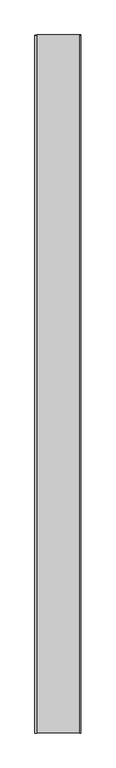
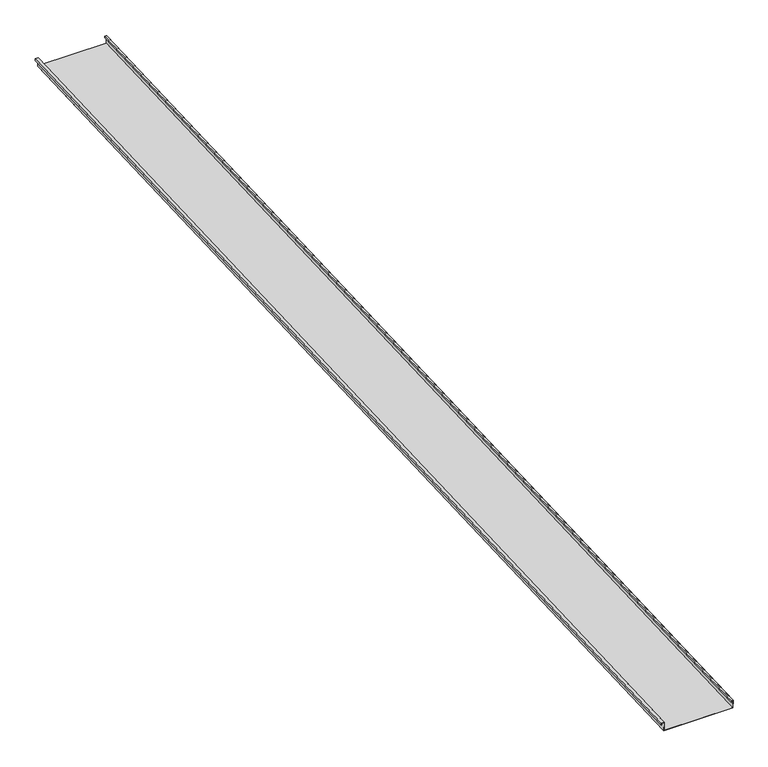
"""IFC4 building model written with IfcOpenShell, lengths in millimetres: proxy geometry, Generic Models 2:Generic Models 2:310765:Generic Models 2:310765 : Generic Models 2:Generic Models 2:310765:121 : Generic Models 2:Generic Models 2:310765:Generic Models 2:310765 : Generic Models 2:Generic Models 2:310765:300385."""

from ifc_helpers import new_model, si_unit, frame, origin, place, context, project, spatial, polyline, outline, extrude, source, transform, mapped, element, save


def generic_models_4ede34d4(model_context):
    return source(origin(), model_context, "Body", "SweptSolid", [
        extrude(outline(polyline([(1.5875, 0.0), (1.5875, 50.8), (407.9875, 50.8), (407.9875, 1.5875), (396.875, 1.5875), (396.875, 11.1125), (398.4625, 11.1125), (398.4625, 3.175), (406.4, 3.175), (406.4, 49.2125), (3.175, 49.2125), (3.175, -1.5874999), (-14.2875, -1.5874999), (-14.2875, 9.525), (-12.7, 9.525), (-12.7, 0.0), (1.5875, 0.0)])), frame((664209.5929738, -581354.4345603, 3902.6697972), z_axis=(0.0, 0.9991330730923568, 0.041630544712067834), x_axis=(1.0, 0.0, 0.0)), (0.0, 0.0, 1.0), 6400.8),
    ])


if __name__ == "__main__":
    model = new_model("IFC4")
    model_context = context("Model", 3, world=origin())
    ifc_project = project(units=[si_unit("LENGTHUNIT", "METRE", prefix="MILLI")], contexts=[model_context])
    site = spatial("IfcSite", under=ifc_project)
    building = spatial("IfcBuilding", under=site)
    placement = place(None, origin())
    generic_models_shape = generic_models_4ede34d4(model_context)
    element("IfcBuildingElementProxy", 1, Name="Generic Models 2:Generic Models 2:310765:Generic Models 2:310765 : Generic Models 2:Generic Models 2:310765:121 : Generic Models 2:Generic Models 2:310765:Generic Models 2:310765 : Generic Models 2:Generic Models 2:310765:300385", ObjectType="Generic Models 2:Generic Models 2:310765:Generic Models 2:310765 : Generic Models 2:Generic Models 2:310765:121 : Generic Models 2:Generic Models 2:310765:Generic Models 2:310765 : Generic Models 2:Generic Models 2:310765:300385", at=placement, inside=building, context=model_context, shape_type="MappedRepresentation", body=[
        mapped(generic_models_shape, transform((0.0, 0.0, 0.0), x_axis=(1.0, 0.0, 0.0), y_axis=(0.0, 1.0, 0.0), z_axis=(0.0, 0.0, 1.0))),
    ])
    save(model, "model.ifc")

# Revit data of these elements
# Type "Generic Models 2:Generic Models 2:310765:Generic Models 2:310765 : Generic Models 2:Generic Models 2:310765:121 : Generic Models 2:Generic Models 2:310765:Generic Models 2:310765 : Generic Models 2:Generic Models 2:310765:300385"
#   NameOverride = "Generic Models 2:Generic Models 2:310765:Generic Models 2:310765 : Generic Models 2:Generic Models 2:310765:300385"
#   ObjectTypeOverride = "Generic Models 2:310765 : Generic Models 2:Generic Models 2:310765"
#   Reference = "Generic Models 2"
#   Tag = "300385"
# Element 1 (IfcBuildingElementProxy, "Generic Models 2:Generic Models 2:310765:Generic Models 2:310765 : Generic Models 2:Generic Models 2:310765:121 : Generic Models 2:Generic Models 2:310765:Generic Models 2:310765 : Generic Models 2:Generic Models 2:310765:300385")
#   Materials on its faces: "THERMAL BROKEN ALUMINUM STOREFRONT FOR POLYCARBONATE"
# Materials
#   "THERMAL BROKEN ALUMINUM STOREFRONT FOR POLYCARBONATE": class "Unassigned", colour RGB 244 244 244, transparency 0, Keynote = "M07611300.01", Cost = 0
